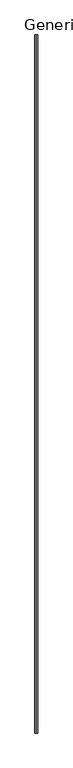
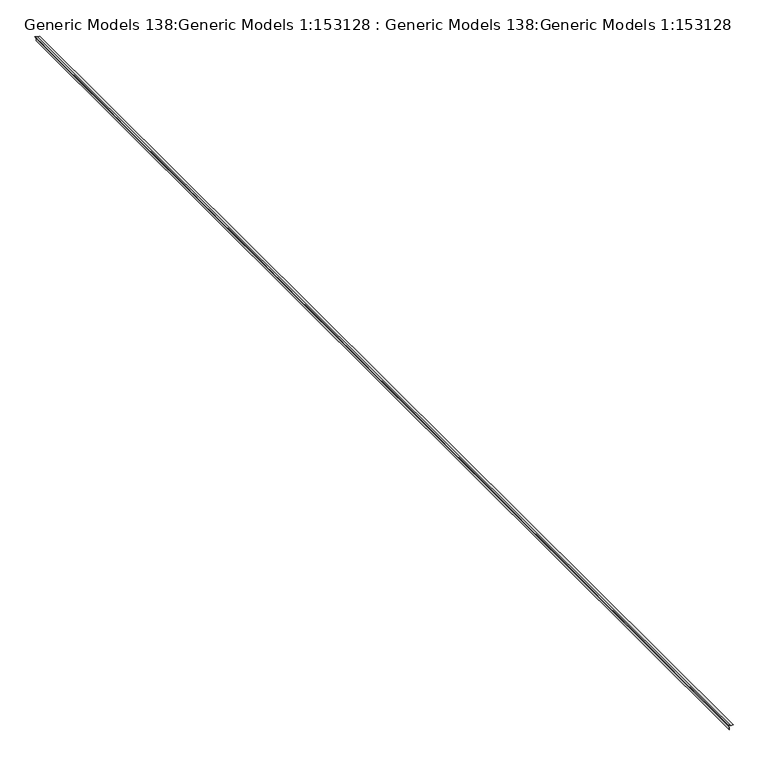
"""IFC4 building model written with IfcOpenShell, lengths in millimetres: proxy geometry, Generic Models 138:Generic Models 1:153128 : Generic Models 138:Generic Models 1:153128."""

from ifc_helpers import new_model, si_unit, point, frame, frame_2d, origin, place, context, project, spatial, polyline, circle_curve, trimmed, segment, composite_curve, outline, extrude, source, transform, mapped, element, save


def generic_models_138_generic_models_1_153128_generic_models_d6e9c702(model_context):
    return source(origin(), model_context, "Body", "SweptSolid", [
        extrude(outline(composite_curve([segment(polyline([(3790.3455135, 7072.6180954), (3809.8721292, 7034.5925808)]), True, "CONTINUOUS"), segment(trimmed(circle_curve(frame_2d((3808.5963009, 7033.9374257)), 1.4342127), [point((3809.8721292, 7034.5925808))], [point((3807.9411458, 7032.6615974))], False, "CARTESIAN"), True, "CONTINUOUS"), segment(polyline([(3807.9411458, 7032.6615974), (3769.9156312, 7052.188213), (3731.8156312, 7052.188213), (3731.8156312, 7053.458213), (3770.2226549, 7053.458213), (3808.9757532, 7033.5579734), (3789.0755135, 7072.3110717), (3789.0755135, 7110.7180954), (3790.3455135, 7110.7180954), (3790.3455135, 7072.6180954)]), True, "CONTINUOUS")], self_intersect=False)), frame((0.0, -6877.9974793, 0.0), z_axis=(0.0, 1.0, 0.0), x_axis=(0.0, 0.0, 1.0)), (0.0, 0.0, 1.0), 19050.0),
    ])


if __name__ == "__main__":
    model = new_model("IFC4")
    model_context = context("Model", 3, world=origin())
    ifc_project = project(units=[si_unit("LENGTHUNIT", "METRE", prefix="MILLI")], contexts=[model_context])
    site = spatial("IfcSite", under=ifc_project)
    building = spatial("IfcBuilding", under=site)
    placement = place(None, origin())
    generic_models_138_generic_models_1_153128_generic_models_shape = generic_models_138_generic_models_1_153128_generic_models_d6e9c702(model_context)
    element("IfcBuildingElementProxy", 1, Name="Generic Models 138:Generic Models 1:153128 : Generic Models 138:Generic Models 1:153128", ObjectType="Generic Models 138:Generic Models 1:153128 : Generic Models 138:Generic Models 1:153128", at=placement, inside=building, context=model_context, shape_type="MappedRepresentation", body=[
        mapped(generic_models_138_generic_models_1_153128_generic_models_shape, transform((0.0, 0.0, 0.0), x_axis=(1.0, 0.0, 0.0), y_axis=(0.0, 1.0, 0.0), z_axis=(0.0, 0.0, 1.0))),
    ])
    save(model, "model.ifc")

# Revit data of these elements
# Type "Generic Models 138:Generic Models 1:153128 : Generic Models 138:Generic Models 1:153128"
#   NameOverride = "Generic Models 138:Generic Models 1:153128"
#   ObjectTypeOverride = "Generic Models 138:Generic Models 1"
#   Reference = "Generic Models 1"
#   Category = "Generic Models"
#   Tag = "153128"
# Element 1 (IfcBuildingElementProxy, "Generic Models 138:Generic Models 1:153128 : Generic Models 138:Generic Models 1:153128")
#   Materials on its faces: "_CONTINUOUS 16 GA. COPPER CORNER BEAD 558"
# Materials
#   "_CONTINUOUS 16 GA. COPPER CORNER BEAD 558": class "Unassigned", colour RGB 253 192 103, transparency 0
